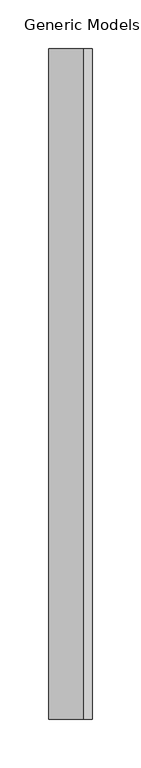
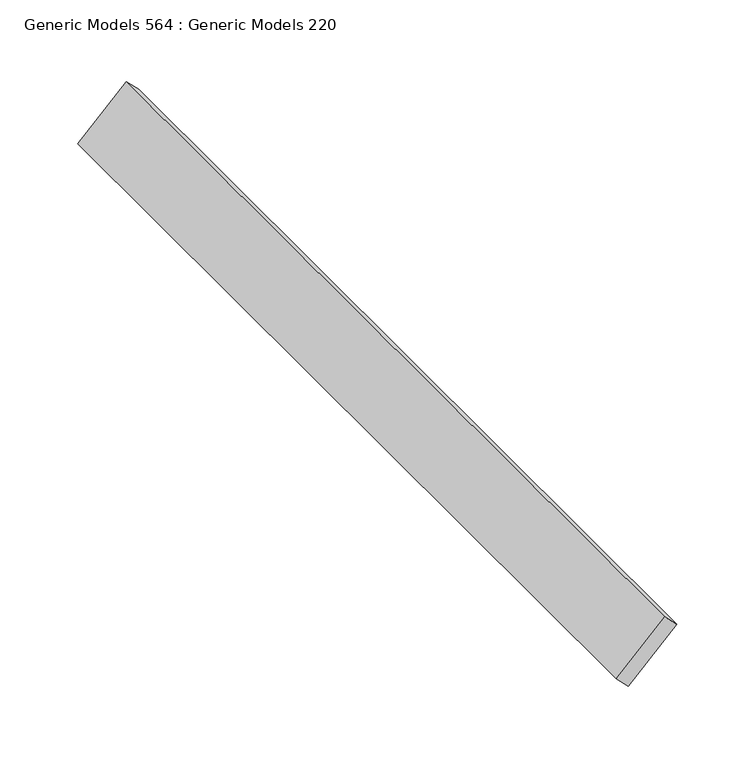
"""IFC4 building model written with IfcOpenShell, lengths in millimetres: proxy geometry, Generic Models 564 : Generic Models 220."""

from ifc_helpers import new_model, si_unit, frame, origin, place, context, project, spatial, polyline, outline, extrude, source, transform, mapped, element, save


def generic_models_564_generic_models_220_bced1f02(model_context):
    return source(origin(), model_context, "Body", "SweptSolid", [
        extrude(outline(polyline([(0.0, -12.7000001), (0.0, 0.0), (690.8142348, 0.0), (690.8142348, -12.7000001), (0.0, -12.7000001)])), frame((7841.3059863, 4539.4872686, 124239.6399101), z_axis=(0.7071067811868034, 0.0, 0.7071067811862918), x_axis=(0.0, -1.0, 0.0)), (0.0, 0.0, 1.0), 50.8),
    ])


if __name__ == "__main__":
    model = new_model("IFC4")
    model_context = context("Model", 3, world=origin())
    ifc_project = project(units=[si_unit("LENGTHUNIT", "METRE", prefix="MILLI")], contexts=[model_context])
    site = spatial("IfcSite", under=ifc_project)
    building = spatial("IfcBuilding", under=site)
    placement = place(None, origin())
    generic_models_564_generic_models_220_shape = generic_models_564_generic_models_220_bced1f02(model_context)
    element("IfcBuildingElementProxy", 1, Name="Generic Models 564 : Generic Models 220", ObjectType="Generic Models 564 : Generic Models 220", at=placement, inside=building, context=model_context, shape_type="MappedRepresentation", body=[
        mapped(generic_models_564_generic_models_220_shape, transform((0.0, 0.0, 0.0), x_axis=(1.0, 0.0, 0.0), y_axis=(0.0, 1.0, 0.0), z_axis=(0.0, 0.0, 1.0))),
    ])
    save(model, "model.ifc")

# Revit data of these elements
# Element 1 (IfcBuildingElementProxy, "Generic Models 564 : Generic Models 220")
#   Materials on its faces: "_WOOD TONE ALUMINUM EXTRUSION SLAT BY KNOTWOOD"
# Materials
#   "_WOOD TONE ALUMINUM EXTRUSION SLAT BY KNOTWOOD": class "Generic", colour RGB 177 130 114, transparency 0, Cost = 0
